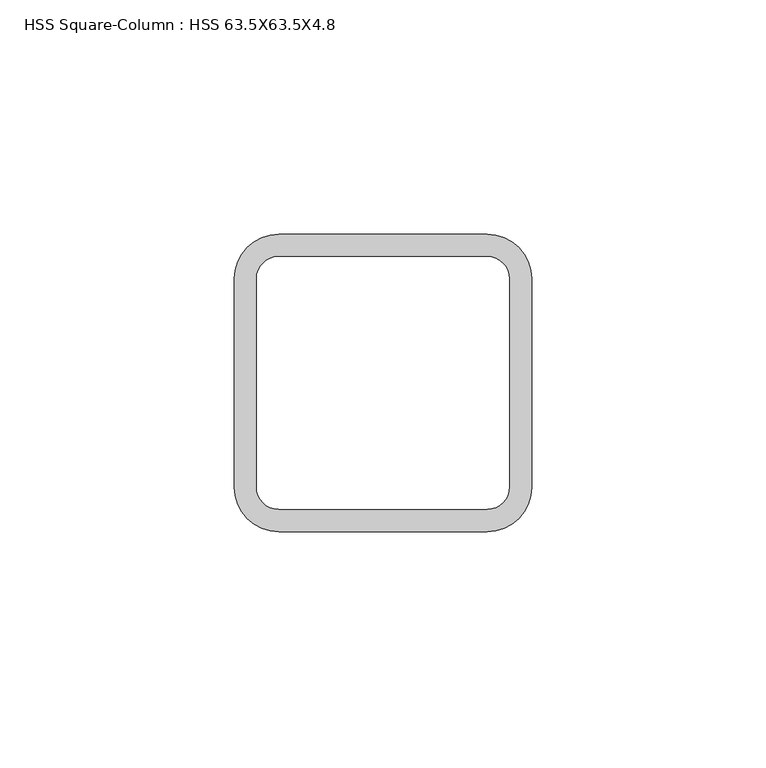
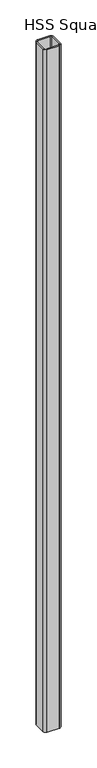
"""IFC4 building model written with IfcOpenShell, lengths in millimetres: column geometry, HSS Square-Column : HSS 63.5X63.5X4.8."""

import ifcopenshell
import ifcopenshell.guid

model = None  # the IFC model being written
_history = None  # IfcOwnerHistory: only IFC2X3 demands one
_inside = {}  # id of a spatial element -> (the spatial element, [elements in it])
_under = {}  # id of a project, library or spatial element -> (it, [spatial elements below it])
_declared = {}  # id of a project -> (the project, [libraries it declares])
_typed = {}  # id of a type object -> (the type object, [elements of that type])
_made_of = {}  # id of a material, layer set ... -> (it, [elements and type objects made of it])


def new_model(schema):
    """Start an empty IFC model of exactly this schema.

    Asked for "IFC4X3", IfcOpenShell would pick the latest addendum, in which some entities
    have other attributes; the version numbers below select the first issue.
    IFC2X3 requires an IfcOwnerHistory on every rooted entity: one is made here for all.
    """
    global model, _history
    if schema == "IFC4X3":
        model = ifcopenshell.file(schema_version=(4, 3, 0, 0))
    else:
        model = ifcopenshell.file(schema=schema)
    _inside.clear()
    _under.clear()
    _declared.clear()
    _typed.clear()
    _made_of.clear()
    _history = None
    if model.schema == "IFC2X3":
        org = make("IfcOrganization", Name="unknown")
        user = make(
            "IfcPersonAndOrganization",
            ThePerson=make("IfcPerson", FamilyName="unknown"),
            TheOrganization=org,
        )
        app = make(
            "IfcApplication",
            ApplicationDeveloper=org,
            Version="unknown",
            ApplicationFullName="unknown",
            ApplicationIdentifier="unknown",
        )
        _history = make(
            "IfcOwnerHistory",
            OwningUser=user,
            OwningApplication=app,
            ChangeAction="ADDED",
            CreationDate=0,
        )
    return model


def make(cls, **values):
    """One entity of the class cls with the attributes given. An attribute that is None is left unset."""
    return model.create_entity(
        cls, **{name: value for name, value in values.items() if value is not None}
    )


def rooted(cls, **values):
    """An entity with a GlobalId (a new one), such as an element, a storey or a relation."""
    return make(cls, GlobalId=ifcopenshell.guid.new(), OwnerHistory=_history, **values)


def si_unit(unit_type, name, prefix=None):
    """IfcSIUnit, for example si_unit("LENGTHUNIT", "METRE", prefix="MILLI")."""
    return make("IfcSIUnit", UnitType=unit_type, Prefix=prefix, Name=name)


def assignment(units):
    """IfcUnitAssignment: the units of a project."""
    return None if units is None else make("IfcUnitAssignment", Units=units)


def point(xyz):
    """IfcCartesianPoint."""
    return None if xyz is None else make("IfcCartesianPoint", Coordinates=xyz)


def direction(xyz):
    """IfcDirection."""
    return None if xyz is None else make("IfcDirection", DirectionRatios=xyz)


def frame(location, z_axis=None, x_axis=None):
    """IfcAxis2Placement3D, a coordinate frame: its origin and axes. An axis left out is left unset."""
    return make(
        "IfcAxis2Placement3D",
        Location=point(location),
        Axis=direction(z_axis),
        RefDirection=direction(x_axis),
    )


def frame_2d(location, x_axis=None):
    """IfcAxis2Placement2D, a coordinate frame in the plane: its origin and x axis."""
    return make(
        "IfcAxis2Placement2D", Location=point(location), RefDirection=direction(x_axis)
    )


def origin():
    """The frame at (0, 0, 0) with its axes left unset."""
    return frame((0.0, 0.0, 0.0))


def place(relative_to, where):
    """IfcLocalPlacement: puts the frame where relative to a parent placement (None: the world)."""
    return make(
        "IfcLocalPlacement", PlacementRelTo=relative_to, RelativePlacement=where
    )


def context(
    kind, dimensions, precision=None, world=None, true_north=None, identifier=None
):
    """IfcGeometricRepresentationContext, for example the 3D "Model" context."""
    return make(
        "IfcGeometricRepresentationContext",
        ContextIdentifier=identifier,
        ContextType=kind,
        CoordinateSpaceDimension=dimensions,
        Precision=precision,
        WorldCoordinateSystem=world,
        TrueNorth=true_north,
    )


def project(units=None, contexts=None):
    """IfcProject with its units and contexts."""
    return rooted(
        "IfcProject",
        Name="project",
        RepresentationContexts=contexts,
        UnitsInContext=assignment(units),
    )


def spatial(cls, under=None, at=None, **own):
    """A site, building, storey or space (cls), placed at a placement, below another one or the project."""
    s = rooted(cls, ObjectPlacement=at, **own)
    if under is not None:
        _under.setdefault(under.id(), (under, []))[1].append(s)
    return s


def polyline(points):
    """IfcPolyline through the points."""
    return make("IfcPolyline", Points=[point(p) for p in points])


def circle_curve(where, radius):
    """IfcCircle in the frame where."""
    return make("IfcCircle", Position=where, Radius=radius)


def trimmed(basis, trim1, trim2, sense, master):
    """IfcTrimmedCurve: the piece of a basis curve between two trims."""
    return make(
        "IfcTrimmedCurve",
        BasisCurve=basis,
        Trim1=trim1,
        Trim2=trim2,
        SenseAgreement=sense,
        MasterRepresentation=master,
    )


def segment(curve, same_sense, transition):
    """IfcCompositeCurveSegment."""
    return make(
        "IfcCompositeCurveSegment",
        Transition=transition,
        SameSense=same_sense,
        ParentCurve=curve,
    )


def composite_curve(segments, self_intersect=None):
    """IfcCompositeCurve: segments joined end to end."""
    return make("IfcCompositeCurve", Segments=segments, SelfIntersect=self_intersect)


def outline(outer, holes=None, kind="AREA"):
    """IfcArbitraryClosedProfileDef: a profile drawn as a closed curve; with holes, ...WithVoids."""
    if holes is None:
        return make("IfcArbitraryClosedProfileDef", ProfileType=kind, OuterCurve=outer)
    return make(
        "IfcArbitraryProfileDefWithVoids",
        ProfileType=kind,
        OuterCurve=outer,
        InnerCurves=holes,
    )


def extrude(swept, where, along, depth):
    """IfcExtrudedAreaSolid: the profile swept, set in the frame where, extruded along a direction by depth."""
    return make(
        "IfcExtrudedAreaSolid",
        SweptArea=swept,
        Position=where,
        ExtrudedDirection=direction(along),
        Depth=depth,
    )


def shape(context_of_items, identifier, shape_type, items):
    """IfcShapeRepresentation: the items that make up one representation, for example the "Body"."""
    return make(
        "IfcShapeRepresentation",
        ContextOfItems=context_of_items,
        RepresentationIdentifier=identifier,
        RepresentationType=shape_type,
        Items=items,
    )


def source(mapping_origin, context_of_items, identifier, shape_type, items):
    """IfcRepresentationMap: a shape defined once, which mapped items show again and again."""
    return make(
        "IfcRepresentationMap",
        MappingOrigin=mapping_origin,
        MappedRepresentation=shape(context_of_items, identifier, shape_type, items),
    )


def transform(
    local_origin,
    x_axis=None,
    y_axis=None,
    z_axis=None,
    scale=None,
    scale2=None,
    scale3=None,
    uniform=True,
):
    """IfcCartesianTransformationOperator3D, or its non-uniform kind. x_axis, y_axis, z_axis: its Axis1, 2, 3."""
    if uniform:
        return make(
            "IfcCartesianTransformationOperator3D",
            Axis1=direction(x_axis),
            Axis2=direction(y_axis),
            LocalOrigin=point(local_origin),
            Scale=scale,
            Axis3=direction(z_axis),
        )
    return make(
        "IfcCartesianTransformationOperator3DnonUniform",
        Axis1=direction(x_axis),
        Axis2=direction(y_axis),
        LocalOrigin=point(local_origin),
        Scale=scale,
        Axis3=direction(z_axis),
        Scale2=scale2,
        Scale3=scale3,
    )


def mapped(mapping_source, mapping_target):
    """IfcMappedItem: shows the shape of a source again, moved by a transform."""
    return make(
        "IfcMappedItem", MappingSource=mapping_source, MappingTarget=mapping_target
    )


def made_of(thing, what):
    """Note that an element or type object is made of a material, layer set ...; save() writes the relation."""
    if what is not None:
        _made_of.setdefault(what.id(), (what, []))[1].append(thing)
    return thing


def element(
    cls,
    number,
    at=None,
    inside=None,
    cuts=None,
    type_object=None,
    material=None,
    context=None,
    identifier="Body",
    shape_type=None,
    held_by="IfcProductDefinitionShape",
    body=None,
    shapes=None,
    **own,
):
    """One element of the class cls, such as IfcWall. Its Tag is "e" and its number.

    at: its placement. inside: the storey or other place that contains it. cuts: it is an
    opening in that element (IfcRelVoidsElement). A single representation is given by context,
    identifier, shape_type and body (its items); several are given by shapes. held_by: the class
    of the entity that holds the representations. save() writes the other relations.
    """
    e = rooted(cls, Tag="e%d" % number, ObjectPlacement=at, **own)
    if body is not None:
        shapes = [shape(context, identifier, shape_type, body)]
    if shapes is not None:
        e.Representation = make(held_by, Representations=shapes)
    if inside is not None:
        _inside.setdefault(inside.id(), (inside, []))[1].append(e)
    if cuts is not None:
        rooted(
            "IfcRelVoidsElement", RelatingBuildingElement=cuts, RelatedOpeningElement=e
        )
    if type_object is not None:
        _typed.setdefault(type_object.id(), (type_object, []))[1].append(e)
    return made_of(e, material)


def aggregate(whole, parts):
    """IfcRelAggregates: a whole, such as a stair, and the parts it consists of."""
    return rooted("IfcRelAggregates", RelatingObject=whole, RelatedObjects=parts)


def save(model, path):
    """Write the relations noted so far, then the file.

    IfcRelAggregates (storeys below a building ...), IfcRelContainedInSpatialStructure (elements
    in a storey), IfcRelDefinesByType, IfcRelAssociatesMaterial and IfcRelDeclares: one each for
    every whole, place, type object, material and project.
    """
    for whole, parts in _under.values():
        aggregate(whole, parts)
    for where, things in _inside.values():
        rooted(
            "IfcRelContainedInSpatialStructure",
            RelatedElements=things,
            RelatingStructure=where,
        )
    for kind, things in _typed.values():
        rooted("IfcRelDefinesByType", RelatedObjects=things, RelatingType=kind)
    for what, things in _made_of.values():
        rooted("IfcRelAssociatesMaterial", RelatedObjects=things, RelatingMaterial=what)
    for by, libraries in _declared.values():
        rooted("IfcRelDeclares", RelatingContext=by, RelatedDefinitions=libraries)
    model.write(path)


def hss_square_column_hss_63_5x63_5x4_8_ac90984b(model_context):
    return source(origin(), model_context, "Body", "SweptSolid", [
        extrude(outline(composite_curve([segment(trimmed(circle_curve(frame_2d((22.225, 22.225)), 9.525), [point((22.225, 31.75))], [point((31.75, 22.225))], False, "CARTESIAN"), True, "CONTINUOUS"), segment(polyline([(31.75, 22.225), (31.75, -22.225)]), True, "CONTINUOUS"), segment(trimmed(circle_curve(frame_2d((22.225, -22.225)), 9.525), [point((31.75, -22.225))], [point((22.225, -31.75))], False, "CARTESIAN"), True, "CONTINUOUS"), segment(polyline([(22.225, -31.75), (-22.225, -31.75)]), True, "CONTINUOUS"), segment(trimmed(circle_curve(frame_2d((-22.225, -22.225)), 9.525), [point((-22.225, -31.75))], [point((-31.75, -22.225))], False, "CARTESIAN"), True, "CONTINUOUS"), segment(polyline([(-31.75, -22.225), (-31.75, 22.225)]), True, "CONTINUOUS"), segment(trimmed(circle_curve(frame_2d((-22.225, 22.225)), 9.525), [point((-31.75, 22.225))], [point((-22.225, 31.75))], False, "CARTESIAN"), True, "CONTINUOUS"), segment(polyline([(-22.225, 31.75), (22.225, 31.75)]), True, "CONTINUOUS")], self_intersect=False), holes=[composite_curve([segment(polyline([(22.225, 26.9875), (-22.225, 26.9875)]), True, "CONTINUOUS"), segment(trimmed(circle_curve(frame_2d((-22.225, 22.225)), 4.7625), [point((-22.225, 26.9875))], [point((-26.9875, 22.225))], True, "CARTESIAN"), True, "CONTINUOUS"), segment(polyline([(-26.9875, 22.225), (-26.9875, -22.225)]), True, "CONTINUOUS"), segment(trimmed(circle_curve(frame_2d((-22.225, -22.225)), 4.7625), [point((-26.9875, -22.225))], [point((-22.225, -26.9875))], True, "CARTESIAN"), True, "CONTINUOUS"), segment(polyline([(-22.225, -26.9875), (22.225, -26.9875)]), True, "CONTINUOUS"), segment(trimmed(circle_curve(frame_2d((22.225, -22.225)), 4.7625), [point((22.225, -26.9875))], [point((26.9875, -22.225))], True, "CARTESIAN"), True, "CONTINUOUS"), segment(polyline([(26.9875, -22.225), (26.9875, 22.225)]), True, "CONTINUOUS"), segment(trimmed(circle_curve(frame_2d((22.225, 22.225)), 4.7625), [point((26.9875, 22.225))], [point((22.225, 26.9875))], True, "CARTESIAN"), True, "CONTINUOUS")], self_intersect=False)]), frame((0.0, 0.0, 6240.0), z_axis=(0.0, 0.0, 1.0), x_axis=(1.0, 0.0, 0.0)), (0.0, 0.0, 1.0), 2650.0),
    ])


if __name__ == "__main__":
    model = new_model("IFC4")
    model_context = context("Model", 3, world=origin())
    ifc_project = project(units=[si_unit("LENGTHUNIT", "METRE", prefix="MILLI")], contexts=[model_context])
    site = spatial("IfcSite", under=ifc_project)
    building = spatial("IfcBuilding", under=site)
    placement = place(None, origin())
    hss_square_column_hss_63_5x63_5x4_8_shape = hss_square_column_hss_63_5x63_5x4_8_ac90984b(model_context)
    element("IfcColumn", 1, ObjectType="HSS Square-Column : HSS 63.5X63.5X4.8", at=placement, inside=building, context=model_context, shape_type="MappedRepresentation", body=[
        mapped(hss_square_column_hss_63_5x63_5x4_8_shape, transform((0.0, 0.0, 0.0), x_axis=(1.0, 0.0, 0.0), y_axis=(0.0, 1.0, 0.0), z_axis=(0.0, 0.0, 1.0))),
    ])
    save(model, "model.ifc")

# Revit data of these elements
# Type "HSS Square-Column : HSS 63.5X63.5X4.8"
#   Section Name Key = "HSS 2 1/2X2 1/2X3/16"
#   Assembly Code = "B10"
#   Width = 6.35 cm
#   Wall Nominal Thickness = 0.4763 cm
#   Wall Design Thickness = 0.442 cm
#   Torsional Moment of Inertia = 93.6521 cm⁴
#   Torsional Modulus = 30.4799 cm³
#   Section Area = 9.93546 cm²
#   Plastic Modulus weak axis = 21.6309 cm³
#   Plastic Modulus strong axis = 21.6309 cm³
#   Outer Fillet = 0.9525 cm
#   Nominal Weight = 8.31884 kgf/m
#   Moment of Inertia weak axis = 56.1912 cm⁴
#   Moment of Inertia strong axis = 56.1912 cm⁴
#   Inner Fillet = 0.4763 cm
#   Height = 6.35 cm
#   Elastic Modulus weak axis = 17.698 cm³
#   Elastic Modulus strong axis = 17.698 cm³
#   Centroid Vertical = 3.175 cm
#   Centroid Horizontal = 3.175 cm
#   Structural Material [instance default] = Steel ASTM A500, Grade B, Rectangular and Square
#   Principal Axes Angle = 0
# Element 1 (IfcColumn, "HSS Square-Column : HSS 63.5X63.5X4.8")
#   Structural Material = none
# Materials
#   "Steel ASTM A500, Grade B, Rectangular and Square": class "Metal", colour RGB 199 199 199, transparency 0, Description = "Carbon steel", Cost = 0
